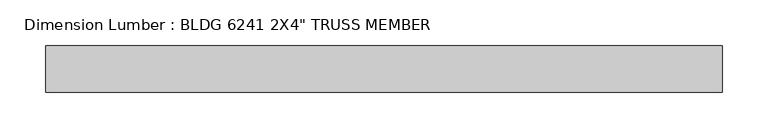
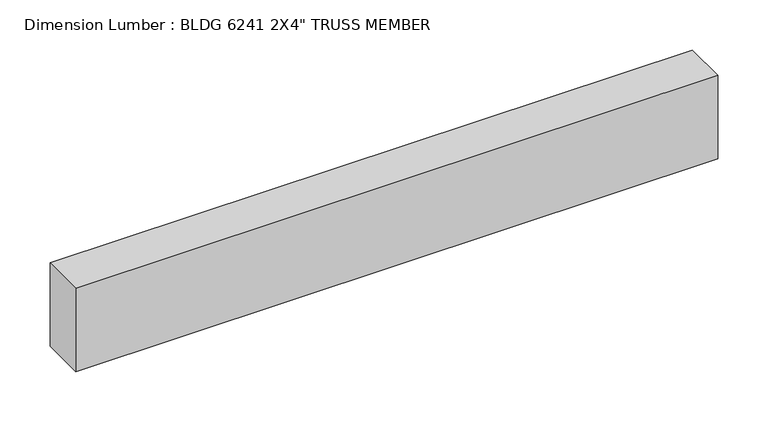
"""IFC4 building model written with IfcOpenShell, lengths in millimetres: beam geometry."""

from ifc_helpers import new_model, si_unit, frame, origin, place, context, project, spatial, polyline, outline, extrude, source, transform, mapped, element, save


def beam_925b2549(model_context):
    return source(origin(), model_context, "Body", "SweptSolid", [
        extrude(outline(polyline([(371.7582386, -25.4), (-368.3, -25.4), (-368.3, 25.4), (371.7582386, 25.4), (371.7582386, -25.4)])), frame((0.0, 0.0, -50.8), z_axis=(0.0, 0.0, 1.0), x_axis=(1.0, 0.0, 0.0)), (0.0, 0.0, 1.0), 101.6),
    ])


if __name__ == "__main__":
    model = new_model("IFC4")
    model_context = context("Model", 3, world=origin())
    ifc_project = project(units=[si_unit("LENGTHUNIT", "METRE", prefix="MILLI")], contexts=[model_context])
    site = spatial("IfcSite", under=ifc_project)
    building = spatial("IfcBuilding", under=site)
    placement = place(None, origin())
    beam_shape = beam_925b2549(model_context)
    element("IfcBeam", 1, ObjectType="Dimension Lumber : BLDG 6241 2X4\" TRUSS MEMBER", at=placement, inside=building, context=model_context, shape_type="MappedRepresentation", body=[
        mapped(beam_shape, transform((0.0, 0.0, 0.0), x_axis=(1.0, 0.0, 0.0), y_axis=(0.0, 1.0, 0.0), z_axis=(0.0, 0.0, 1.0))),
    ])
    save(model, "model.ifc")

# Revit data of these elements
# Type "Dimension Lumber : BLDG 6241 2X4\" TRUSS MEMBER"
#   Assembly Code = "B10"
#   A = 0.273472 SF
#   Length [instance default] = 5' - 0"
#   b = 0' - 2"
#   d = 0' - 4"
#   Structural Material [instance default] = Softwood, Lumber
# Element 1 (IfcBeam, "Dimension Lumber : BLDG 6241 2X4\" TRUSS MEMBER")
#   Materials on its faces: "Softwood, Lumber"
# Materials
#   "Softwood, Lumber": class "Wood", colour RGB 223 192 134, transparency 0, Description = "Pinus Echinata", Cost = 0
